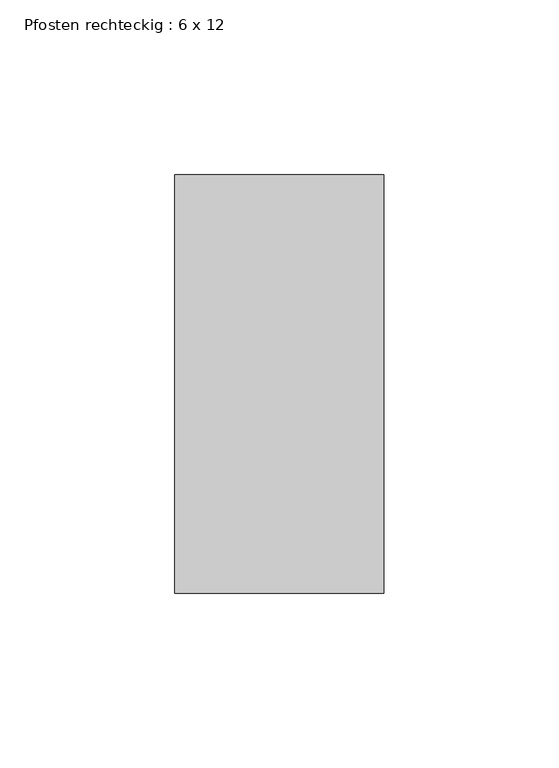
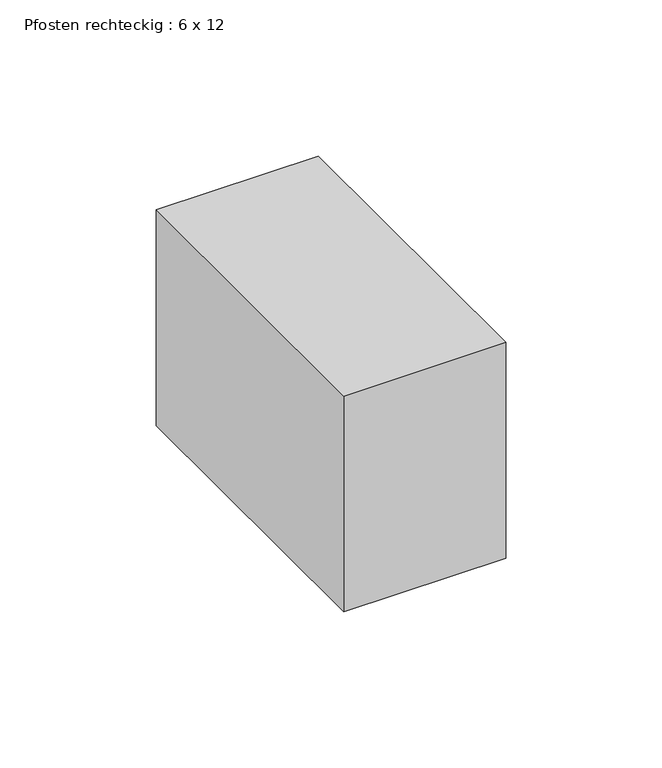
"""IFC4 building model written with IfcOpenShell, lengths in millimetres: member geometry, Pfosten rechteckig : 6 x 12."""

from ifc_helpers import new_model, si_unit, frame, origin, place, context, project, spatial, polyline, outline, extrude, source, transform, mapped, element, save


def pfosten_rechteckig_6_x_12_3e976124(model_context):
    return source(origin(), model_context, "Body", "SweptSolid", [
        extrude(outline(polyline([(30.0, 60.0), (30.0, -60.0), (-30.0, -60.0), (-30.0, 60.0), (30.0, 60.0)])), frame((0.0, 0.0, -84.3558419), z_axis=(0.0, 0.0, 1.0), x_axis=(1.0, 0.0, 0.0)), (0.0, 0.0, 1.0), 84.3558419),
    ])


if __name__ == "__main__":
    model = new_model("IFC4")
    model_context = context("Model", 3, world=origin())
    ifc_project = project(units=[si_unit("LENGTHUNIT", "METRE", prefix="MILLI")], contexts=[model_context])
    site = spatial("IfcSite", under=ifc_project)
    building = spatial("IfcBuilding", under=site)
    placement = place(None, origin())
    pfosten_rechteckig_6_x_12_shape = pfosten_rechteckig_6_x_12_3e976124(model_context)
    element("IfcMember", 1, ObjectType="Pfosten rechteckig : 6 x 12", at=placement, inside=building, context=model_context, shape_type="MappedRepresentation", body=[
        mapped(pfosten_rechteckig_6_x_12_shape, transform((0.0, 0.0, 0.0), x_axis=(1.0, 0.0, 0.0), y_axis=(0.0, 1.0, 0.0), z_axis=(0.0, 0.0, 1.0))),
    ])
    save(model, "model.ifc")

# Revit data of these elements
# Type "Pfosten rechteckig : 6 x 12"
#   built-in parameter 1007304 = 0.393701 (stored number, unit not read)
#   built-in parameter 1007301 = 0.0984252 (stored number, unit not read)
#   built-in parameter 1007300 = 0.0984252 (stored number, unit not read)
# Element 1 (IfcMember, "Pfosten rechteckig : 6 x 12")
#   Materials on its faces: "Metall - verzinkt"
# Materials
#   "Metall - verzinkt": class "Allgemeines", colour RGB 200 200 200, transparency 0, Cost = 0
